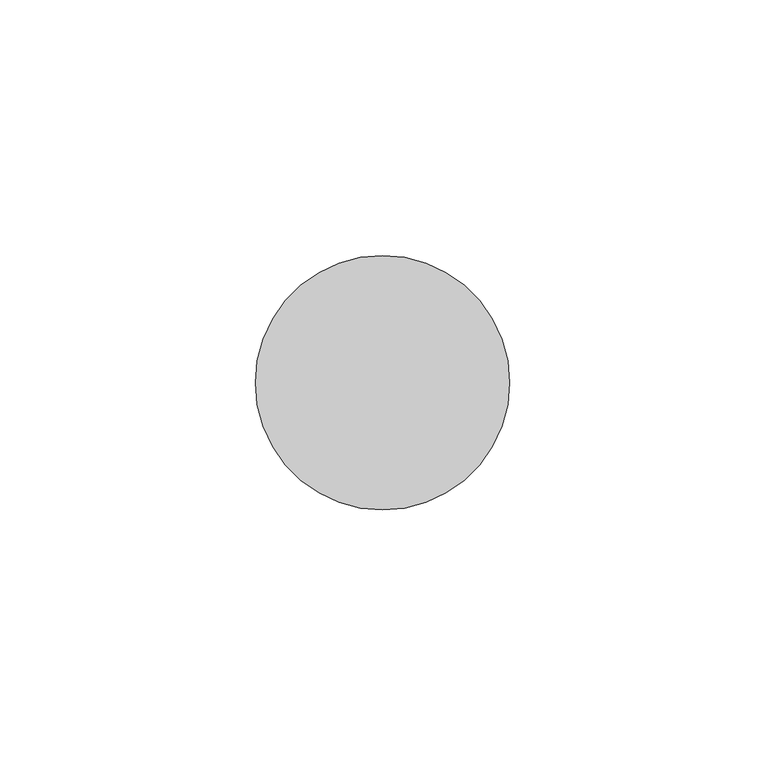
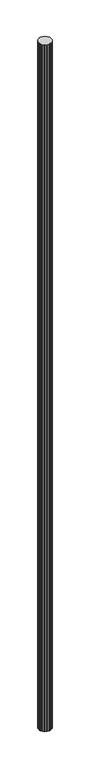
"""IFC4 building model written with IfcOpenShell, lengths in millimetres: proxy geometry, 0_3d."""

from ifc_helpers import new_model, si_unit, origin, origin_with_axes, place, context, project, spatial, polyline, outline, extrude, source, transform, mapped, element, save


def generic_models_b6edaf92(model_context):
    return source(origin(), model_context, "Body", "SweptSolid", [
        extrude(outline(polyline([(49.5185707, 29.3232855), (49.8968091, 25.0), (49.5185707, 20.6767145), (48.3953478, 16.4847898), (46.5612692, 12.5515954), (44.0720623, 8.9966396), (41.0033604, 5.9279377), (37.4484046, 3.4387308), (33.5152102, 1.6046522), (29.3232855, 0.4814293), (25.0, 0.1031909), (20.6767145, 0.4814293), (16.4847898, 1.6046522), (12.5515954, 3.4387308), (8.9966396, 5.9279377), (5.9279377, 8.9966396), (3.4387308, 12.5515954), (1.6046522, 16.4847898), (0.4814293, 20.6767145), (0.1031909, 25.0), (0.4814293, 29.3232855), (1.6046522, 33.5152102), (3.4387308, 37.4484046), (5.9279377, 41.0033604), (8.9966396, 44.0720623), (12.5515954, 46.5612692), (16.4847898, 48.3953478), (20.6767145, 49.5185707), (25.0, 49.8968091), (29.3232855, 49.5185707), (33.5152102, 48.3953478), (37.4484046, 46.5612692), (41.0033604, 44.0720623), (44.0720623, 41.0033604), (46.5612692, 37.4484046), (48.3953478, 33.5152102), (49.5185707, 29.3232855)])), origin_with_axes(), (0.0, 0.0, 1.0), 2855.0),
    ])


if __name__ == "__main__":
    model = new_model("IFC4")
    model_context = context("Model", 3, world=origin())
    ifc_project = project(units=[si_unit("LENGTHUNIT", "METRE", prefix="MILLI")], contexts=[model_context])
    site = spatial("IfcSite", under=ifc_project)
    building = spatial("IfcBuilding", under=site)
    placement = place(None, origin())
    generic_models_shape = generic_models_b6edaf92(model_context)
    element("IfcBuildingElementProxy", 1, Name="0_3d", ObjectType="0_3d", at=placement, inside=building, context=model_context, shape_type="MappedRepresentation", body=[
        mapped(generic_models_shape, transform((0.0, 0.0, 0.0), x_axis=(1.0, 0.0, 0.0), y_axis=(0.0, 1.0, 0.0), z_axis=(0.0, 0.0, 1.0))),
    ])
    save(model, "model.ifc")

# Revit data of these elements
# Element 1 (IfcBuildingElementProxy, "0_3d")
#   Materials on its faces: "alu"
# Materials
#   "alu": class "Unassigned", colour RGB 219 219 219, transparency 0
